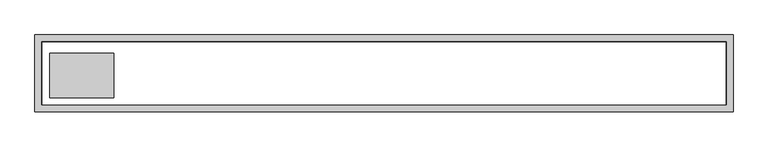
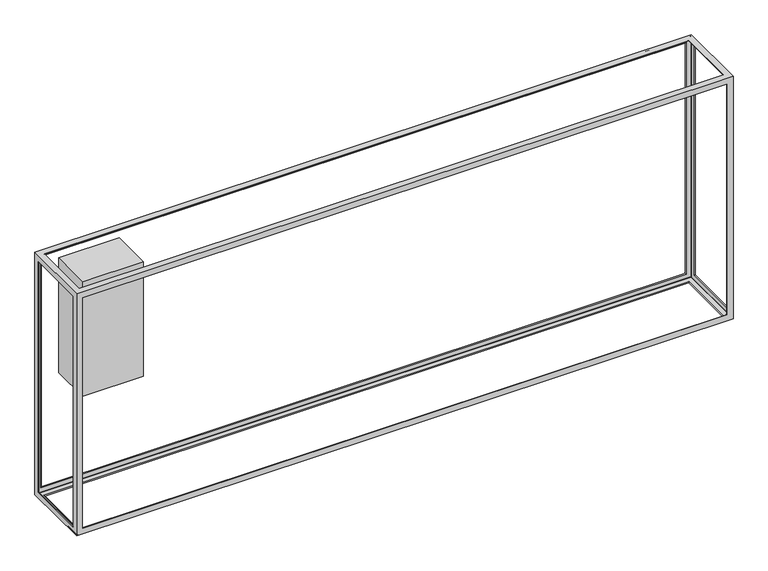
"""IFC4 building model written with IfcOpenShell, lengths in millimetres: beam geometry, Plumbing Bulkhead : EX. BULKHEAD 1 (MODIFIED)."""

from ifc_helpers import new_model, si_unit, frame, origin, place, context, project, spatial, polyline, ellipse_curve, outline, extrude, source, transform, mapped, element, save
from ifc_brep_helpers import plane_surface, cylinder_surface, revolved_surface, advanced_brep


def beam_e0c467be(model_context):
    return source(origin(), model_context, "Body", "SolidModel", [
        extrude(outline(polyline([(379.0365927, 279.4), (379.0365927, 66.5145898), (70.4236299, 66.5145898), (70.4236299, 279.4), (379.0365927, 279.4)])), frame((0.0, 0.0, 688.452765), z_axis=(0.0, 0.0, 1.0), x_axis=(1.0, 0.0, 0.0)), (0.0, 0.0, 1.0), 619.647235),
        advanced_brep(
        [(0.0, 0.0, 1308.1), (0.0, 368.3, 1308.1), (0.0, 368.3, 0.0), (0.0, 0.0, 0.0), (0.0, 31.75, 1276.35), (0.0, 31.75, 31.75), (0.0, 336.55, 31.75), (0.0, 336.55, 1276.35), (3352.8, 368.3, 1308.1), (3352.8, 368.3, 0.0), (3321.05, 368.3, 31.75), (3321.05, 368.3, 1276.35), (31.75, 368.3, 1276.35), (31.75, 368.3, 31.75), (3352.8, 0.0, 0.0), (3321.05, 336.55, 0.0), (31.75, 336.55, 0.0), (31.75, 31.75, 0.0), (3321.05, 31.75, 0.0), (3352.8, 0.0, 1308.1), (3321.05, 0.0, 1276.35), (3321.05, 0.0, 31.75), (31.75, 0.0, 31.75), (31.75, 0.0, 1276.35), (3.175, 28.575, 1279.525), (3.175, 28.575, 28.575), (3.175, 339.725, 28.575), (3.175, 339.725, 1279.525), (3352.8, 336.55, 31.75), (3349.625, 339.725, 28.575), (3349.625, 28.575, 28.575), (3352.8, 31.75, 31.75), (3352.8, 31.75, 1276.35), (3352.8, 336.55, 1276.35), (3349.625, 28.575, 1279.525), (3349.625, 339.725, 1279.525), (3324.225, 339.725, 3.175), (28.575, 339.725, 3.175), (28.575, 28.575, 3.175), (3324.225, 28.575, 3.175), (3348.0375, 4.7625, 3.175), (3348.0375, 363.5375, 3.175), (4.7625, 363.5375, 3.175), (4.7625, 4.7625, 3.175), (3349.160032, 364.660032, 3.639968), (3349.160032, 3.639968, 3.639968), (3349.625, 4.7625, 4.7625), (3349.625, 363.5375, 4.7625), (3348.0375, 365.125, 4.7625), (4.7625, 365.125, 4.7625), (3.639968, 364.660032, 3.639968), (3.175, 363.5375, 4.7625), (3.175, 4.7625, 4.7625), (3.639968, 3.639968, 3.639968), (4.7625, 3.175, 4.7625), (3348.0375, 3.175, 4.7625), (3348.0375, 365.125, 1303.3375), (4.7625, 365.125, 1303.3375), (3324.225, 365.125, 1279.525), (3324.225, 365.125, 28.575), (28.575, 365.125, 28.575), (28.575, 365.125, 1279.525), (3.639968, 364.660032, 1304.460032), (3.175, 363.5375, 1303.3375), (3349.625, 363.5375, 1303.3375), (3349.160032, 364.660032, 1304.460032), (3349.625, 4.7625, 1303.3375), (3348.0375, 3.175, 1303.3375), (3349.160032, 3.639968, 1304.460032), (3.175, 4.7625, 1303.3375), (4.7625, 3.175, 1303.3375), (3.639968, 3.639968, 1304.460032), (3324.225, 3.175, 1279.525), (3324.225, 3.175, 28.575), (28.575, 3.175, 28.575), (28.575, 3.175, 1279.525), (31.75, 31.75, 1308.1), (31.75, 336.55, 1308.1), (3321.05, 336.55, 1308.1), (3321.05, 31.75, 1308.1), (28.575, 339.725, 1304.925), (3324.225, 339.725, 1304.925), (4.7625, 4.7625, 1304.925), (4.7625, 363.5375, 1304.925), (3348.0375, 363.5375, 1304.925), (3348.0375, 4.7625, 1304.925), (28.575, 28.575, 1304.925), (3324.225, 28.575, 1304.925)],
        [
            (0, 1),
            (1, 2),
            (2, 3),
            (3, 0),
            (4, 5),
            (5, 6),
            (6, 7),
            (7, 4),
            (8, 9),
            (9, 2),
            (1, 8),
            (10, 11),
            (11, 12),
            (12, 13),
            (13, 10),
            (9, 14),
            (14, 3),
            (15, 16),
            (16, 17),
            (17, 18),
            (18, 15),
            (14, 19),
            (19, 0),
            (20, 21),
            (21, 22),
            (22, 23),
            (23, 20),
            (4, 24, ellipse_curve(frame((0.0, 28.575, 1279.525), z_axis=(0.0, -0.7071067811865464, -0.7071067811865487), x_axis=(0.0, 0.7071067811865487, -0.7071067811865464)), 4.4901281, 3.175)),
            (24, 25),
            (25, 5, ellipse_curve(frame((0.0, 28.575, 28.575), z_axis=(0.0, -0.7071067811865499, 0.7071067811865451), x_axis=(0.0, -0.7071067811865451, -0.7071067811865498)), 4.4901281, 3.175)),
            (25, 26),
            (26, 6, ellipse_curve(frame((0.0, 339.725, 28.575), z_axis=(0.0, -0.707106781186545, -0.70710678118655), x_axis=(0.0, -0.7071067811865501, 0.7071067811865449)), 4.4901281, 3.175)),
            (27, 7, ellipse_curve(frame((0.0, 339.725, 1279.525), z_axis=(0.0, 0.7071067811865487, -0.7071067811865464), x_axis=(0.0, -0.7071067811865465, -0.7071067811865487)), 4.4901281, 3.175)),
            (26, 27),
            (28, 29, ellipse_curve(frame((3352.8, 339.725, 28.575), z_axis=(0.0, -0.7071067811865429, -0.7071067811865522), x_axis=(0.0, -0.7071067811865521, 0.707106781186543)), 4.4901281, 3.175)),
            (29, 30),
            (30, 31, ellipse_curve(frame((3352.8, 28.575, 28.575), z_axis=(0.0, 0.7071067811865499, -0.7071067811865451), x_axis=(0.0, -0.7071067811865451, -0.70710678118655)), 4.4901281, 3.175)),
            (31, 28),
            (8, 19),
            (31, 32),
            (32, 33),
            (33, 28),
            (30, 34),
            (34, 32, ellipse_curve(frame((3352.8, 28.575, 1279.525), z_axis=(0.0, -0.7071067811865464, -0.7071067811865487), x_axis=(0.0, 0.7071067811865487, -0.7071067811865464)), 4.4901281, 3.175)),
            (33, 35, ellipse_curve(frame((3352.8, 339.725, 1279.525), z_axis=(0.0, 0.7071067811865509, -0.7071067811865441), x_axis=(0.0, -0.707106781186544, -0.7071067811865509)), 4.4901281, 3.175)),
            (35, 29),
            (15, 36, ellipse_curve(frame((3324.225, 339.725, 0.0), z_axis=(-0.7071067811865475, 0.7071067811865475, 0.0), x_axis=(-0.7071067811865476, -0.7071067811865474, 0.0)), 4.4901281, 3.175)),
            (36, 37),
            (37, 16, ellipse_curve(frame((28.575, 339.725, 0.0), z_axis=(0.7071067811865454, 0.7071067811865498, 0.0), x_axis=(-0.7071067811865497, 0.7071067811865454, 0.0)), 4.4901281, 3.175)),
            (37, 38),
            (38, 17, ellipse_curve(frame((28.575, 28.575, 0.0), z_axis=(-0.7071067811865498, 0.7071067811865452, 0.0), x_axis=(-0.7071067811865451, -0.7071067811865498, 0.0)), 4.4901281, 3.175)),
            (39, 18, ellipse_curve(frame((3324.225, 28.575, 0.0), z_axis=(-0.7071067811865475, -0.7071067811865475, 0.0), x_axis=(-0.7071067811865476, 0.7071067811865474, 0.0)), 4.4901281, 3.175)),
            (38, 39),
            (39, 36),
            (40, 41),
            (41, 42),
            (42, 43),
            (43, 40),
            (44, 41, ellipse_curve(frame((3348.0375, 363.5375, 4.7625), z_axis=(-0.7071067811865475, 0.7071067811865475, 0.0), x_axis=(0.7071067811865474, 0.7071067811865476, 0.0)), 2.245064, 1.5875)),
            (40, 45, ellipse_curve(frame((3348.0375, 4.7625, 4.7625), z_axis=(-0.7071067811865475, -0.7071067811865475, 0.0), x_axis=(-0.7071067811865474, 0.7071067811865476, 0.0)), 2.245064, 1.5875)),
            (45, 46, ellipse_curve(frame((3348.0375, 4.7625, 4.7625), z_axis=(0.0, -0.7071067811865499, 0.7071067811865451), x_axis=(0.0, 0.7071067811865451, 0.70710678118655)), 2.245064, 1.5875)),
            (46, 47),
            (47, 44, ellipse_curve(frame((3348.0375, 363.5375, 4.7625), z_axis=(0.0, 0.7071067811865429, 0.7071067811865522), x_axis=(0.0, 0.7071067811865521, -0.707106781186543)), 2.245064, 1.5875)),
            (48, 49),
            (49, 50, ellipse_curve(frame((4.7625, 363.5375, 4.7625), z_axis=(-0.7071067811865439, 0.0, 0.7071067811865511), x_axis=(0.7071067811865511, 0.0, 0.7071067811865438)), 2.245064, 1.5875)),
            (50, 42, ellipse_curve(frame((4.7625, 363.5375, 4.7625), z_axis=(-0.7071067811865454, -0.7071067811865498, 0.0), x_axis=(0.7071067811865497, -0.7071067811865454, 0.0)), 2.245064, 1.5875)),
            (44, 48, ellipse_curve(frame((3348.0375, 363.5375, 4.7625), z_axis=(0.7071067811865475, 0.0, 0.7071067811865476), x_axis=(0.7071067811865475, 0.0, -0.7071067811865475)), 2.245064, 1.5875)),
            (51, 52),
            (52, 53, ellipse_curve(frame((4.7625, 4.7625, 4.7625), z_axis=(0.0, -0.7071067811865499, 0.7071067811865451), x_axis=(0.0, 0.7071067811865451, 0.70710678118655)), 2.245064, 1.5875)),
            (53, 43, ellipse_curve(frame((4.7625, 4.7625, 4.7625), z_axis=(0.7071067811865498, -0.7071067811865452, 0.0), x_axis=(0.7071067811865451, 0.7071067811865498, 0.0)), 2.245064, 1.5875)),
            (50, 51, ellipse_curve(frame((4.7625, 363.5375, 4.7625), z_axis=(0.0, 0.707106781186545, 0.70710678118655), x_axis=(0.0, 0.7071067811865501, -0.7071067811865449)), 2.245064, 1.5875)),
            (53, 54, ellipse_curve(frame((4.7625, 4.7625, 4.7625), z_axis=(-0.7071067811865439, 0.0, 0.7071067811865511), x_axis=(0.7071067811865511, 0.0, 0.7071067811865438)), 2.245064, 1.5875)),
            (54, 55),
            (55, 45, ellipse_curve(frame((3348.0375, 4.7625, 4.7625), z_axis=(0.7071067811865475, 0.0, 0.7071067811865476), x_axis=(0.7071067811865475, 0.0, -0.7071067811865475)), 2.245064, 1.5875)),
            (48, 56),
            (56, 57),
            (57, 49),
            (58, 59),
            (59, 60),
            (60, 61),
            (61, 58),
            (57, 62, ellipse_curve(frame((4.7625, 363.5375, 1303.3375), z_axis=(0.7071067811865511, 0.0, 0.7071067811865439), x_axis=(-0.7071067811865438, 0.0, 0.7071067811865511)), 2.245064, 1.5875)),
            (62, 63, ellipse_curve(frame((4.7625, 363.5375, 1303.3375), z_axis=(0.0, -0.7071067811865487, 0.7071067811865464), x_axis=(0.0, 0.7071067811865465, 0.7071067811865487)), 2.245064, 1.5875)),
            (63, 51),
            (47, 64),
            (64, 65, ellipse_curve(frame((3348.0375, 363.5375, 1303.3375), z_axis=(0.0, -0.7071067811865509, 0.7071067811865441), x_axis=(0.0, 0.707106781186544, 0.7071067811865509)), 2.245064, 1.5875)),
            (65, 56, ellipse_curve(frame((3348.0375, 363.5375, 1303.3375), z_axis=(-0.7071067811865475, 0.0, 0.7071067811865475), x_axis=(0.7071067811865474, 0.0, 0.7071067811865476)), 2.245064, 1.5875)),
            (10, 59, ellipse_curve(frame((3324.225, 368.3, 28.575), z_axis=(0.7071067811865475, 0.0, 0.7071067811865476), x_axis=(0.7071067811865476, 0.0, -0.7071067811865475)), 4.4901281, 3.175)),
            (58, 11, ellipse_curve(frame((3324.225, 368.3, 1279.525), z_axis=(0.7071067811865475, 0.0, -0.7071067811865475), x_axis=(-0.7071067811865474, 0.0, -0.7071067811865476)), 4.4901281, 3.175)),
            (13, 60, ellipse_curve(frame((28.575, 368.3, 28.575), z_axis=(0.7071067811865439, 0.0, -0.7071067811865511), x_axis=(-0.7071067811865511, 0.0, -0.7071067811865438)), 4.4901281, 3.175)),
            (12, 61, ellipse_curve(frame((28.575, 368.3, 1279.525), z_axis=(-0.7071067811865511, 0.0, -0.7071067811865439), x_axis=(0.7071067811865438, 0.0, -0.7071067811865511)), 4.4901281, 3.175)),
            (46, 66),
            (66, 64),
            (35, 34),
            (55, 67),
            (67, 68, ellipse_curve(frame((3348.0375, 4.7625, 1303.3375), z_axis=(-0.7071067811865475, 0.0, 0.7071067811865475), x_axis=(0.7071067811865474, 0.0, 0.7071067811865476)), 2.245064, 1.5875)),
            (68, 66, ellipse_curve(frame((3348.0375, 4.7625, 1303.3375), z_axis=(0.0, 0.7071067811865464, 0.7071067811865487), x_axis=(0.0, -0.7071067811865487, 0.7071067811865464)), 2.245064, 1.5875)),
            (63, 69),
            (69, 52),
            (24, 27),
            (70, 54),
            (69, 71, ellipse_curve(frame((4.7625, 4.7625, 1303.3375), z_axis=(0.0, 0.7071067811865464, 0.7071067811865487), x_axis=(0.0, -0.7071067811865487, 0.7071067811865464)), 2.245064, 1.5875)),
            (71, 70, ellipse_curve(frame((4.7625, 4.7625, 1303.3375), z_axis=(0.7071067811865511, 0.0, 0.7071067811865439), x_axis=(-0.7071067811865438, 0.0, 0.7071067811865511)), 2.245064, 1.5875)),
            (72, 73),
            (73, 21, ellipse_curve(frame((3324.225, 0.0, 28.575), z_axis=(0.7071067811865475, 0.0, 0.7071067811865476), x_axis=(0.7071067811865476, 0.0, -0.7071067811865475)), 4.4901281, 3.175)),
            (20, 72, ellipse_curve(frame((3324.225, 0.0, 1279.525), z_axis=(0.7071067811865475, 0.0, -0.7071067811865475), x_axis=(-0.7071067811865474, 0.0, -0.7071067811865476)), 4.4901281, 3.175)),
            (73, 74),
            (74, 22, ellipse_curve(frame((28.575, 0.0, 28.575), z_axis=(0.7071067811865439, 0.0, -0.7071067811865511), x_axis=(-0.7071067811865511, 0.0, -0.7071067811865438)), 4.4901281, 3.175)),
            (74, 75),
            (75, 23, ellipse_curve(frame((28.575, 0.0, 1279.525), z_axis=(-0.7071067811865511, 0.0, -0.7071067811865439), x_axis=(0.7071067811865438, 0.0, -0.7071067811865511)), 4.4901281, 3.175)),
            (70, 67),
            (72, 75),
            (76, 77),
            (77, 78),
            (78, 79),
            (79, 76),
            (77, 80, ellipse_curve(frame((28.575, 339.725, 1308.1), z_axis=(0.707106781186548, 0.7071067811865469, 0.0), x_axis=(-0.707106781186547, 0.7071067811865478, 0.0)), 4.4901281, 3.175)),
            (80, 81),
            (81, 78, ellipse_curve(frame((3324.225, 339.725, 1308.1), z_axis=(-0.7071067811865469, 0.707106781186548, 0.0), x_axis=(-0.7071067811865481, -0.7071067811865468, 0.0)), 4.4901281, 3.175)),
            (82, 83),
            (83, 84),
            (84, 85),
            (85, 82),
            (80, 86),
            (86, 87),
            (87, 81),
            (65, 84, ellipse_curve(frame((3348.0375, 363.5375, 1303.3375), z_axis=(0.7071067811865469, -0.707106781186548, 0.0), x_axis=(0.7071067811865481, 0.7071067811865468, 0.0)), 2.245064, 1.5875)),
            (83, 62, ellipse_curve(frame((4.7625, 363.5375, 1303.3375), z_axis=(-0.707106781186548, -0.7071067811865469, 0.0), x_axis=(0.707106781186547, -0.7071067811865478, 0.0)), 2.245064, 1.5875)),
            (86, 76, ellipse_curve(frame((28.575, 28.575, 1308.1), z_axis=(0.7071067811865469, -0.707106781186548, 0.0), x_axis=(-0.7071067811865481, -0.7071067811865468, 0.0)), 4.4901281, 3.175)),
            (79, 87, ellipse_curve(frame((3324.225, 28.575, 1308.1), z_axis=(-0.707106781186548, -0.7071067811865469, 0.0), x_axis=(-0.707106781186547, 0.7071067811865478, 0.0)), 4.4901281, 3.175)),
            (71, 82, ellipse_curve(frame((4.7625, 4.7625, 1303.3375), z_axis=(-0.7071067811865469, 0.707106781186548, 0.0), x_axis=(0.7071067811865481, 0.7071067811865468, 0.0)), 2.245064, 1.5875)),
            (85, 68, ellipse_curve(frame((3348.0375, 4.7625, 1303.3375), z_axis=(0.707106781186548, 0.7071067811865469, 0.0), x_axis=(0.707106781186547, -0.7071067811865478, 0.0)), 2.245064, 1.5875)),
        ],
        [
            plane_surface(frame((0.0, 368.3, 0.0), z_axis=(-1.0, 0.0, 0.0), x_axis=(0.0, 0.0, 1.0))),
            plane_surface(frame((0.0, 368.3, 31.75), z_axis=(0.0, 1.0, 0.0), x_axis=(1.0, 0.0, 0.0))),
            plane_surface(frame((0.0, 368.3, 0.0), z_axis=(0.0, 0.0, -1.0), x_axis=(1.0, 0.0, 0.0))),
            plane_surface(frame((3352.8, 0.0, 0.0), z_axis=(0.0, -1.0, 0.0), x_axis=(0.0, 0.0, 1.0))),
            cylinder_surface(frame((0.0, 28.575, 0.0), z_axis=(0.0, 0.0, -1.0), x_axis=(0.0, 1.0, 0.0)), 3.175),
            cylinder_surface(frame((0.0, 0.0, 28.575), z_axis=(0.0, -1.0, 0.0), x_axis=(1.0, 0.0, 0.0)), 3.175),
            cylinder_surface(frame((0.0, 339.725, 0.0), z_axis=(0.0, 0.0, -1.0), x_axis=(0.0, -1.0, 0.0)), 3.175),
            cylinder_surface(frame((3352.8, 0.0, 28.575), z_axis=(0.0, -1.0, 0.0), x_axis=(-1.0, 0.0, 0.0)), 3.175),
            plane_surface(frame((3352.8, 368.3, 0.0), z_axis=(1.0, 0.0, 0.0), x_axis=(0.0, 0.0, 1.0))),
            cylinder_surface(frame((3352.8, 28.575, 0.0), z_axis=(0.0, 0.0, -1.0), x_axis=(0.0, 1.0, 0.0)), 3.175),
            cylinder_surface(frame((3352.8, 339.725, 0.0), z_axis=(0.0, 0.0, -1.0), x_axis=(0.0, -1.0, 0.0)), 3.175),
            cylinder_surface(frame((0.0, 339.725, 0.0), z_axis=(-1.0, 0.0, 0.0), x_axis=(0.0, -1.0, 0.0)), 3.175),
            cylinder_surface(frame((28.575, 0.0, 0.0), z_axis=(0.0, -1.0, 0.0), x_axis=(1.0, 0.0, 0.0)), 3.175),
            cylinder_surface(frame((0.0, 28.575, 0.0), z_axis=(-1.0, 0.0, 0.0), x_axis=(0.0, 1.0, 0.0)), 3.175),
            cylinder_surface(frame((3324.225, 0.0, 0.0), z_axis=(0.0, -1.0, 0.0), x_axis=(-1.0, 0.0, 0.0)), 3.175),
            plane_surface(frame((0.0, 339.725, 3.175), z_axis=(0.0, 0.0, 1.0), x_axis=(1.0, 0.0, 0.0))),
            revolved_surface(polyline([(3346.45, 365.1249999785978, 4.7625), (3346.45, 3.1750000214022047, 4.7625)]), (3348.0375, 0.0, 4.7625), (0.0, 1.0, 0.0)),
            revolved_surface(polyline([(3349.6249999785978, 361.95000000000005, 4.7625), (3.175000021402197, 361.95000000000005, 4.7625)]), (0.0, 363.5375, 4.7625), (1.0, 0.0, 0.0)),
            revolved_surface(polyline([(6.35, 365.1249999785978, 4.7625), (6.35, 3.1750000214022, 4.7625)]), (4.7625, 0.0, 4.7625), (0.0, 1.0, 0.0)),
            revolved_surface(polyline([(3349.6249999785978, 6.35, 4.7625), (3.175000021402197, 6.35, 4.7625)]), (0.0, 4.7625, 4.7625), (1.0, 0.0, 0.0)),
            plane_surface(frame((0.0, 365.125, 4.7625), z_axis=(0.0, -1.0, 0.0), x_axis=(1.0, 0.0, 0.0))),
            revolved_surface(polyline([(4.7625, 361.95000000000005, 1304.924999978598), (4.7625, 361.95000000000005, 3.1750000214022105)]), (4.7625, 363.5375, 0.0), (0.0, 0.0, 1.0)),
            revolved_surface(polyline([(3348.0375, 361.95000000000005, 1304.924999978598), (3348.0375, 361.95000000000005, 3.175000021402205)]), (3348.0375, 363.5375, 0.0), (0.0, 0.0, 1.0)),
            cylinder_surface(frame((3324.225, 368.3, 0.0), z_axis=(0.0, 0.0, -1.0), x_axis=(0.0, -1.0, 0.0)), 3.175),
            cylinder_surface(frame((0.0, 368.3, 28.575), z_axis=(-1.0, 0.0, 0.0), x_axis=(0.0, -1.0, 0.0)), 3.175),
            cylinder_surface(frame((28.575, 368.3, 0.0), z_axis=(0.0, 0.0, -1.0), x_axis=(0.0, -1.0, 0.0)), 3.175),
            plane_surface(frame((3349.625, 339.725, 0.0), z_axis=(-1.0, 0.0, 0.0), x_axis=(0.0, 0.0, 1.0))),
            revolved_surface(polyline([(3348.0375, 6.35, 1304.924999978598), (3348.0375, 6.35, 3.1750000214021994)]), (3348.0375, 4.7625, 0.0), (0.0, 0.0, 1.0)),
            plane_surface(frame((3.175, 363.5375, 0.0), z_axis=(1.0, 0.0, 0.0), x_axis=(0.0, 0.0, 1.0))),
            revolved_surface(polyline([(4.7625, 6.35, 1304.924999978598), (4.7625, 6.35, 3.1750000214021994)]), (4.7625, 4.7625, 0.0), (0.0, 0.0, 1.0)),
            cylinder_surface(frame((3324.225, 0.0, 0.0), z_axis=(0.0, 0.0, -1.0), x_axis=(0.0, 1.0, 0.0)), 3.175),
            cylinder_surface(frame((0.0, 0.0, 28.575), z_axis=(-1.0, 0.0, 0.0), x_axis=(0.0, 1.0, 0.0)), 3.175),
            cylinder_surface(frame((28.575, 0.0, 0.0), z_axis=(0.0, 0.0, -1.0), x_axis=(0.0, 1.0, 0.0)), 3.175),
            plane_surface(frame((0.0, 3.175, 1303.3375), z_axis=(0.0, 1.0, 0.0), x_axis=(1.0, 0.0, 0.0))),
            plane_surface(frame((3352.8, 368.3, 1308.1), z_axis=(0.0, 0.0, 1.0), x_axis=(1.0, 0.0, 0.0))),
            cylinder_surface(frame((0.0, 339.725, 1308.1), z_axis=(-1.0, 0.0, 0.0), x_axis=(0.0, -1.0, 0.0)), 3.175),
            plane_surface(frame((0.0, 363.5375, 1304.925), z_axis=(0.0, 0.0, -1.0), x_axis=(1.0, 0.0, 0.0))),
            revolved_surface(polyline([(3349.6249999785978, 361.95000000000005, 1303.3375), (3.175000021402206, 361.95000000000005, 1303.3375)]), (0.0, 363.5375, 1303.3375), (1.0, 0.0, 0.0)),
            cylinder_surface(frame((0.0, 368.3, 1279.525), z_axis=(-1.0, 0.0, 0.0), x_axis=(0.0, -1.0, 0.0)), 3.175),
            cylinder_surface(frame((0.0, 28.575, 1308.1), z_axis=(-1.0, 0.0, 0.0), x_axis=(0.0, 1.0, 0.0)), 3.175),
            revolved_surface(polyline([(3349.6249999785978, 6.35, 1303.3375), (3.1750000214022034, 6.35, 1303.3375)]), (0.0, 4.7625, 1303.3375), (1.0, 0.0, 0.0)),
            cylinder_surface(frame((0.0, 0.0, 1279.525), z_axis=(-1.0, 0.0, 0.0), x_axis=(0.0, 1.0, 0.0)), 3.175),
            cylinder_surface(frame((28.575, 0.0, 1308.1), z_axis=(0.0, -1.0, 0.0), x_axis=(1.0, 0.0, 0.0)), 3.175),
            revolved_surface(polyline([(6.35, 365.1249999785978, 1303.3375), (6.35, 3.1750000214022025, 1303.3375)]), (4.7625, 0.0, 1303.3375), (0.0, 1.0, 0.0)),
            cylinder_surface(frame((0.0, 0.0, 1279.525), z_axis=(0.0, -1.0, 0.0), x_axis=(1.0, 0.0, 0.0)), 3.175),
            cylinder_surface(frame((3324.225, 0.0, 1308.1), z_axis=(0.0, -1.0, 0.0), x_axis=(-1.0, 0.0, 0.0)), 3.175),
            revolved_surface(polyline([(3346.45, 365.1249999785978, 1303.3375), (3346.45, 3.1750000214022025, 1303.3375)]), (3348.0375, 0.0, 1303.3375), (0.0, 1.0, 0.0)),
            cylinder_surface(frame((3352.8, 0.0, 1279.525), z_axis=(0.0, -1.0, 0.0), x_axis=(-1.0, 0.0, 0.0)), 3.175),
        ],
        [
            (0, [[1, 2, 3, 4], [5, 6, 7, 8]]),
            (1, [[9, 10, -2, 11], [12, 13, 14, 15]]),
            (2, [[-3, -10, 16, 17], [18, 19, 20, 21]]),
            (3, [[-17, 22, 23, -4], [24, 25, 26, 27]]),
            (4, [[28, 29, 30, -5]]),
            (5, [[31, 32, -6, -30]]),
            (6, [[33, -7, -32, 34]]),
            (7, [[35, 36, 37, 38]]),
            (8, [[-16, -9, 39, -22], [-38, 40, 41, 42]]),
            (9, [[-37, 43, 44, -40]]),
            (10, [[-35, -42, 45, 46]]),
            (11, [[47, 48, 49, -18]]),
            (12, [[-19, -49, 50, 51]]),
            (13, [[52, -20, -51, 53]]),
            (14, [[-47, -21, -52, 54]]),
            (15, [[55, 56, 57, 58], [-54, -53, -50, -48]]),
            (16, [[59, -55, 60, 61, 62, 63]]),
            (17, [[64, 65, 66, -56, -59, 67]]),
            (18, [[68, 69, 70, -57, -66, 71]]),
            (19, [[-60, -58, -70, 72, 73, 74]]),
            (20, [[75, 76, 77, -64], [78, 79, 80, 81]]),
            (21, [[-77, 82, 83, 84, -71, -65]]),
            (22, [[-75, -67, -63, 85, 86, 87]]),
            (23, [[88, -78, 89, -12]]),
            (24, [[-88, -15, 90, -79]]),
            (25, [[-80, -90, -14, 91]]),
            (26, [[-62, 92, 93, -85], [-36, -46, 94, -43]]),
            (27, [[-61, -74, 95, 96, 97, -92]]),
            (28, [[98, 99, -68, -84], [100, -34, -31, -29]]),
            (29, [[101, -72, -69, -99, 102, 103]]),
            (30, [[104, 105, -24, 106]]),
            (31, [[-105, 107, 108, -25]]),
            (32, [[109, 110, -26, -108]]),
            (33, [[-95, -73, -101, 111], [-104, 112, -109, -107]]),
            (34, [[-1, -23, -39, -11], [113, 114, 115, 116]]),
            (35, [[117, 118, 119, -114]]),
            (36, [[120, 121, 122, 123], [124, 125, 126, -118]]),
            (37, [[-76, -87, 127, -121, 128, -82]]),
            (38, [[-89, -81, -91, -13]]),
            (39, [[129, -116, 130, -125]]),
            (40, [[-111, -103, 131, -123, 132, -96]]),
            (41, [[-106, -27, -110, -112]]),
            (42, [[-113, -129, -124, -117]]),
            (43, [[-128, -120, -131, -102, -98, -83]]),
            (44, [[-8, -33, -100, -28]]),
            (45, [[-126, -130, -115, -119]]),
            (46, [[-86, -93, -97, -132, -122, -127]]),
            (47, [[-41, -44, -94, -45]]),
        ],
    ),
    ])


if __name__ == "__main__":
    model = new_model("IFC4")
    model_context = context("Model", 3, world=origin())
    ifc_project = project(units=[si_unit("LENGTHUNIT", "METRE", prefix="MILLI")], contexts=[model_context])
    site = spatial("IfcSite", under=ifc_project)
    building = spatial("IfcBuilding", under=site)
    placement = place(None, origin())
    beam_shape = beam_e0c467be(model_context)
    element("IfcBeam", 1, ObjectType="Plumbing Bulkhead : EX. BULKHEAD 1 (MODIFIED)", at=placement, inside=building, context=model_context, shape_type="MappedRepresentation", body=[
        mapped(beam_shape, transform((0.0, 0.0, 0.0), x_axis=(1.0, 0.0, 0.0), y_axis=(0.0, 1.0, 0.0), z_axis=(0.0, 0.0, 1.0))),
    ])
    save(model, "model.ifc")

# Revit data of these elements
# Type "Plumbing Bulkhead : EX. BULKHEAD 1 (MODIFIED)"
#   Length = 11' - 0"
#   Height = 4' - 3 1/2"
#   Depth = 1' - 2 1/2"
#   Structural Material = USE EXISTING BULKHEADS IN STORAGE (MODIFY AS NECESSARY)
#   EP MATERIAL = ELECTRICAL PANEL
# Element 1 (IfcBeam, "Plumbing Bulkhead : EX. BULKHEAD 1 (MODIFIED)")
#   Materials on its faces: "USE EXISTING BULKHEADS IN STORAGE (MODIFY AS NECESSARY)", "ELECTRICAL PANEL"
# Materials
#   "USE EXISTING BULKHEADS IN STORAGE (MODIFY AS NECESSARY)": class "Generic", colour RGB 120 120 120, transparency 0, Cost = 0
#   "ELECTRICAL PANEL": class "Generic", colour RGB 255 255 255, transparency 0, Cost = 0
